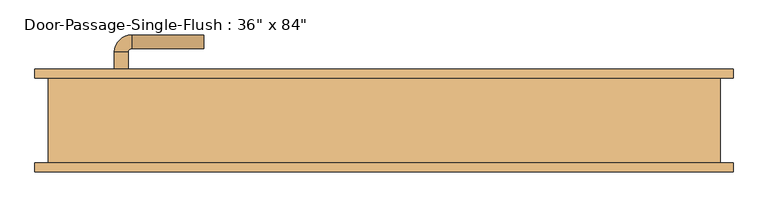
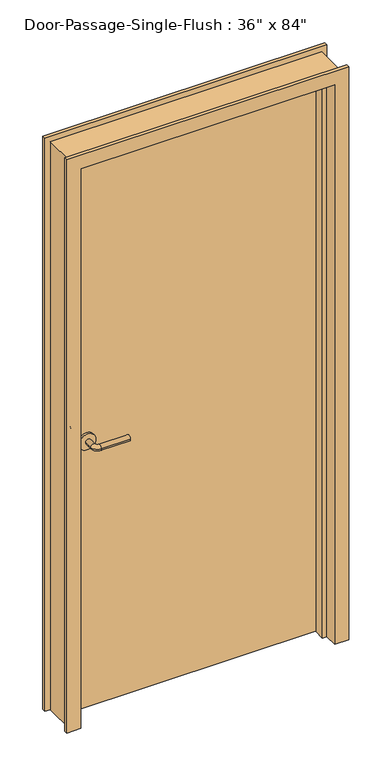
"""IFC4 building model written with IfcOpenShell, lengths in millimetres: door geometry."""

import ifcopenshell
import ifcopenshell.guid

model = None  # the IFC model being written
_history = None  # IfcOwnerHistory: only IFC2X3 demands one
_inside = {}  # id of a spatial element -> (the spatial element, [elements in it])
_under = {}  # id of a project, library or spatial element -> (it, [spatial elements below it])
_declared = {}  # id of a project -> (the project, [libraries it declares])
_typed = {}  # id of a type object -> (the type object, [elements of that type])
_made_of = {}  # id of a material, layer set ... -> (it, [elements and type objects made of it])


def new_model(schema):
    """Start an empty IFC model of exactly this schema.

    Asked for "IFC4X3", IfcOpenShell would pick the latest addendum, in which some entities
    have other attributes; the version numbers below select the first issue.
    IFC2X3 requires an IfcOwnerHistory on every rooted entity: one is made here for all.
    """
    global model, _history
    if schema == "IFC4X3":
        model = ifcopenshell.file(schema_version=(4, 3, 0, 0))
    else:
        model = ifcopenshell.file(schema=schema)
    _inside.clear()
    _under.clear()
    _declared.clear()
    _typed.clear()
    _made_of.clear()
    _history = None
    if model.schema == "IFC2X3":
        org = make("IfcOrganization", Name="unknown")
        user = make(
            "IfcPersonAndOrganization",
            ThePerson=make("IfcPerson", FamilyName="unknown"),
            TheOrganization=org,
        )
        app = make(
            "IfcApplication",
            ApplicationDeveloper=org,
            Version="unknown",
            ApplicationFullName="unknown",
            ApplicationIdentifier="unknown",
        )
        _history = make(
            "IfcOwnerHistory",
            OwningUser=user,
            OwningApplication=app,
            ChangeAction="ADDED",
            CreationDate=0,
        )
    return model


def make(cls, **values):
    """One entity of the class cls with the attributes given. An attribute that is None is left unset."""
    return model.create_entity(
        cls, **{name: value for name, value in values.items() if value is not None}
    )


def rooted(cls, **values):
    """An entity with a GlobalId (a new one), such as an element, a storey or a relation."""
    return make(cls, GlobalId=ifcopenshell.guid.new(), OwnerHistory=_history, **values)


def si_unit(unit_type, name, prefix=None):
    """IfcSIUnit, for example si_unit("LENGTHUNIT", "METRE", prefix="MILLI")."""
    return make("IfcSIUnit", UnitType=unit_type, Prefix=prefix, Name=name)


def assignment(units):
    """IfcUnitAssignment: the units of a project."""
    return None if units is None else make("IfcUnitAssignment", Units=units)


def point(xyz):
    """IfcCartesianPoint."""
    return None if xyz is None else make("IfcCartesianPoint", Coordinates=xyz)


def direction(xyz):
    """IfcDirection."""
    return None if xyz is None else make("IfcDirection", DirectionRatios=xyz)


def frame(location, z_axis=None, x_axis=None):
    """IfcAxis2Placement3D, a coordinate frame: its origin and axes. An axis left out is left unset."""
    return make(
        "IfcAxis2Placement3D",
        Location=point(location),
        Axis=direction(z_axis),
        RefDirection=direction(x_axis),
    )


def frame_2d(location, x_axis=None):
    """IfcAxis2Placement2D, a coordinate frame in the plane: its origin and x axis."""
    return make(
        "IfcAxis2Placement2D", Location=point(location), RefDirection=direction(x_axis)
    )


def origin():
    """The frame at (0, 0, 0) with its axes left unset."""
    return frame((0.0, 0.0, 0.0))


def origin_with_axes():
    """The frame at (0, 0, 0) with the z axis (0, 0, 1) and the x axis (1, 0, 0) written out."""
    return frame((0.0, 0.0, 0.0), z_axis=(0.0, 0.0, 1.0), x_axis=(1.0, 0.0, 0.0))


def place(relative_to, where):
    """IfcLocalPlacement: puts the frame where relative to a parent placement (None: the world)."""
    return make(
        "IfcLocalPlacement", PlacementRelTo=relative_to, RelativePlacement=where
    )


def context(
    kind, dimensions, precision=None, world=None, true_north=None, identifier=None
):
    """IfcGeometricRepresentationContext, for example the 3D "Model" context."""
    return make(
        "IfcGeometricRepresentationContext",
        ContextIdentifier=identifier,
        ContextType=kind,
        CoordinateSpaceDimension=dimensions,
        Precision=precision,
        WorldCoordinateSystem=world,
        TrueNorth=true_north,
    )


def project(units=None, contexts=None):
    """IfcProject with its units and contexts."""
    return rooted(
        "IfcProject",
        Name="project",
        RepresentationContexts=contexts,
        UnitsInContext=assignment(units),
    )


def spatial(cls, under=None, at=None, **own):
    """A site, building, storey or space (cls), placed at a placement, below another one or the project."""
    s = rooted(cls, ObjectPlacement=at, **own)
    if under is not None:
        _under.setdefault(under.id(), (under, []))[1].append(s)
    return s


def polyline(points):
    """IfcPolyline through the points."""
    return make("IfcPolyline", Points=[point(p) for p in points])


def circle_curve(where, radius):
    """IfcCircle in the frame where."""
    return make("IfcCircle", Position=where, Radius=radius)


def ellipse_curve(where, semi_axis1, semi_axis2):
    """IfcEllipse in the frame where."""
    return make(
        "IfcEllipse", Position=where, SemiAxis1=semi_axis1, SemiAxis2=semi_axis2
    )


def trimmed(basis, trim1, trim2, sense, master):
    """IfcTrimmedCurve: the piece of a basis curve between two trims."""
    return make(
        "IfcTrimmedCurve",
        BasisCurve=basis,
        Trim1=trim1,
        Trim2=trim2,
        SenseAgreement=sense,
        MasterRepresentation=master,
    )


def segment(curve, same_sense, transition):
    """IfcCompositeCurveSegment."""
    return make(
        "IfcCompositeCurveSegment",
        Transition=transition,
        SameSense=same_sense,
        ParentCurve=curve,
    )


def composite_curve(segments, self_intersect=None):
    """IfcCompositeCurve: segments joined end to end."""
    return make("IfcCompositeCurve", Segments=segments, SelfIntersect=self_intersect)


def outline(outer, holes=None, kind="AREA"):
    """IfcArbitraryClosedProfileDef: a profile drawn as a closed curve; with holes, ...WithVoids."""
    if holes is None:
        return make("IfcArbitraryClosedProfileDef", ProfileType=kind, OuterCurve=outer)
    return make(
        "IfcArbitraryProfileDefWithVoids",
        ProfileType=kind,
        OuterCurve=outer,
        InnerCurves=holes,
    )


def extrude(swept, where, along, depth):
    """IfcExtrudedAreaSolid: the profile swept, set in the frame where, extruded along a direction by depth."""
    return make(
        "IfcExtrudedAreaSolid",
        SweptArea=swept,
        Position=where,
        ExtrudedDirection=direction(along),
        Depth=depth,
    )


def faces_of(points, faces, orient=None, outer=None):
    """IfcFace entities. A face is a list of loops; a loop is a list of indices into points, from 0.

    orient and outer hold one flag for each loop. By default every Orientation is true, the
    first loop of a face is its IfcFaceOuterBound and the others are IfcFaceBound.
    """
    made = []
    for i, loops in enumerate(faces):
        bounds = []
        for j, loop in enumerate(loops):
            is_outer = j == 0 if outer is None else outer[i][j]
            bounds.append(
                make(
                    "IfcFaceOuterBound" if is_outer else "IfcFaceBound",
                    Bound=make("IfcPolyLoop", Polygon=[points[k] for k in loop]),
                    Orientation=True if orient is None else orient[i][j],
                )
            )
        made.append(make("IfcFace", Bounds=bounds))
    return made


def faceted_brep(points, faces, orient=None, outer=None, voids=None):
    """IfcFacetedBrep: a solid bounded by flat faces; with voids (closed shells), ...WithVoids."""
    shared = [point(p) for p in points]
    hull = make("IfcClosedShell", CfsFaces=faces_of(shared, faces, orient, outer))
    if voids is None:
        return make("IfcFacetedBrep", Outer=hull)
    return make(
        "IfcFacetedBrepWithVoids",
        Outer=hull,
        Voids=[
            make(cls, CfsFaces=faces_of(shared, fs, o, b)) for cls, fs, o, b in voids
        ],
    )


def shape(context_of_items, identifier, shape_type, items):
    """IfcShapeRepresentation: the items that make up one representation, for example the "Body"."""
    return make(
        "IfcShapeRepresentation",
        ContextOfItems=context_of_items,
        RepresentationIdentifier=identifier,
        RepresentationType=shape_type,
        Items=items,
    )


def source(mapping_origin, context_of_items, identifier, shape_type, items):
    """IfcRepresentationMap: a shape defined once, which mapped items show again and again."""
    return make(
        "IfcRepresentationMap",
        MappingOrigin=mapping_origin,
        MappedRepresentation=shape(context_of_items, identifier, shape_type, items),
    )


def transform(
    local_origin,
    x_axis=None,
    y_axis=None,
    z_axis=None,
    scale=None,
    scale2=None,
    scale3=None,
    uniform=True,
):
    """IfcCartesianTransformationOperator3D, or its non-uniform kind. x_axis, y_axis, z_axis: its Axis1, 2, 3."""
    if uniform:
        return make(
            "IfcCartesianTransformationOperator3D",
            Axis1=direction(x_axis),
            Axis2=direction(y_axis),
            LocalOrigin=point(local_origin),
            Scale=scale,
            Axis3=direction(z_axis),
        )
    return make(
        "IfcCartesianTransformationOperator3DnonUniform",
        Axis1=direction(x_axis),
        Axis2=direction(y_axis),
        LocalOrigin=point(local_origin),
        Scale=scale,
        Axis3=direction(z_axis),
        Scale2=scale2,
        Scale3=scale3,
    )


def mapped(mapping_source, mapping_target):
    """IfcMappedItem: shows the shape of a source again, moved by a transform."""
    return make(
        "IfcMappedItem", MappingSource=mapping_source, MappingTarget=mapping_target
    )


def made_of(thing, what):
    """Note that an element or type object is made of a material, layer set ...; save() writes the relation."""
    if what is not None:
        _made_of.setdefault(what.id(), (what, []))[1].append(thing)
    return thing


def element(
    cls,
    number,
    at=None,
    inside=None,
    cuts=None,
    type_object=None,
    material=None,
    context=None,
    identifier="Body",
    shape_type=None,
    held_by="IfcProductDefinitionShape",
    body=None,
    shapes=None,
    **own,
):
    """One element of the class cls, such as IfcWall. Its Tag is "e" and its number.

    at: its placement. inside: the storey or other place that contains it. cuts: it is an
    opening in that element (IfcRelVoidsElement). A single representation is given by context,
    identifier, shape_type and body (its items); several are given by shapes. held_by: the class
    of the entity that holds the representations. save() writes the other relations.
    """
    e = rooted(cls, Tag="e%d" % number, ObjectPlacement=at, **own)
    if body is not None:
        shapes = [shape(context, identifier, shape_type, body)]
    if shapes is not None:
        e.Representation = make(held_by, Representations=shapes)
    if inside is not None:
        _inside.setdefault(inside.id(), (inside, []))[1].append(e)
    if cuts is not None:
        rooted(
            "IfcRelVoidsElement", RelatingBuildingElement=cuts, RelatedOpeningElement=e
        )
    if type_object is not None:
        _typed.setdefault(type_object.id(), (type_object, []))[1].append(e)
    return made_of(e, material)


def aggregate(whole, parts):
    """IfcRelAggregates: a whole, such as a stair, and the parts it consists of."""
    return rooted("IfcRelAggregates", RelatingObject=whole, RelatedObjects=parts)


def save(model, path):
    """Write the relations noted so far, then the file.

    IfcRelAggregates (storeys below a building ...), IfcRelContainedInSpatialStructure (elements
    in a storey), IfcRelDefinesByType, IfcRelAssociatesMaterial and IfcRelDeclares: one each for
    every whole, place, type object, material and project.
    """
    for whole, parts in _under.values():
        aggregate(whole, parts)
    for where, things in _inside.values():
        rooted(
            "IfcRelContainedInSpatialStructure",
            RelatedElements=things,
            RelatingStructure=where,
        )
    for kind, things in _typed.values():
        rooted("IfcRelDefinesByType", RelatedObjects=things, RelatingType=kind)
    for what, things in _made_of.values():
        rooted("IfcRelAssociatesMaterial", RelatedObjects=things, RelatingMaterial=what)
    for by, libraries in _declared.values():
        rooted("IfcRelDeclares", RelatingContext=by, RelatedDefinitions=libraries)
    model.write(path)


def plane_surface(at):
    """IfcPlane: the flat surface through the origin of the frame at, square to its z axis."""
    return make("IfcPlane", Position=at)


def cylinder_surface(at, radius):
    """IfcCylindricalSurface: all points at the distance radius from the z axis of the frame at."""
    return make("IfcCylindricalSurface", Position=at, Radius=radius)


def revolved_surface(curve, axis_point, axis_direction):
    """IfcSurfaceOfRevolution: the curve turned about the line through axis_point along axis_direction."""
    return make(
        "IfcSurfaceOfRevolution",
        SweptCurve=make("IfcArbitraryOpenProfileDef", ProfileType="CURVE", Curve=curve),
        AxisPosition=make("IfcAxis1Placement", Location=point(axis_point), Axis=direction(axis_direction)),
    )


def advanced_brep(points, edges, surfaces, faces):
    """IfcAdvancedBrep: a solid bounded by faces that lie on surfaces and meet in shared edges.

    An edge is (start, end): straight between two places in points (the first is 0);
    or (start, end, curve); or (start, end, curve, False) where it runs against its curve.
    A face is (place in surfaces, loops), or (place, loops, False) where it looks against
    its surface's normal. A loop lists edges by number (the first is 1), with a minus sign
    where the edge is run from its end to its start. The first loop is the outer one.
    """
    corners = [point(p) for p in points]
    vertices = [make("IfcVertexPoint", VertexGeometry=c) for c in corners]
    made = []
    for start, end, *more in edges:
        made.append(
            make(
                "IfcEdgeCurve",
                EdgeStart=vertices[start],
                EdgeEnd=vertices[end],
                EdgeGeometry=more[0] if more else make("IfcPolyline", Points=[corners[start], corners[end]]),
                SameSense=more[1] if len(more) > 1 else True,
            )
        )
    hull = []
    for where, loops, *sense in faces:
        bounds = []
        for j, loop in enumerate(loops):
            ring = [make("IfcOrientedEdge", EdgeElement=made[abs(k) - 1], Orientation=k > 0) for k in loop]
            bounds.append(
                make(
                    "IfcFaceOuterBound" if j == 0 else "IfcFaceBound",
                    Bound=make("IfcEdgeLoop", EdgeList=ring),
                    Orientation=True,
                )
            )
        hull.append(make("IfcAdvancedFace", Bounds=bounds, FaceSurface=surfaces[where], SameSense=sense[0] if sense else True))
    return make("IfcAdvancedBrep", Outer=make("IfcClosedShell", CfsFaces=hull))


def door_6d6a07ab(model_context):
    return source(origin(), model_context, "Body", "SolidModel", [
        advanced_brep(
        [(-392.190625, 15.8125, 1016.0), (-372.190625, 15.8125, 1016.0), (-372.190625, -14.1875, 1016.0), (-392.190625, -14.1875, 1016.0), (-367.190625, -19.1875, 1016.0), (-367.190625, -39.1875, 1016.0), (-262.190625, -39.1875, 1016.0), (-262.190625, -19.1875, 1016.0)],
        [
            (0, 1, circle_curve(frame((-382.190625, 15.8125, 1016.0), z_axis=(0.0, 1.0, 0.0), x_axis=(1.0, 0.0, 0.0)), 10.0)),
            (1, 0, circle_curve(frame((-382.190625, 15.8125, 1016.0), z_axis=(0.0, 1.0, 0.0), x_axis=(1.0, 0.0, 0.0)), 10.0)),
            (1, 2),
            (2, 3, circle_curve(frame((-382.190625, -14.1875, 1016.0), z_axis=(0.0, 1.0, 0.0), x_axis=(1.0, 0.0, 0.0)), 10.0)),
            (3, 0),
            (3, 2, circle_curve(frame((-382.190625, -14.1875, 1016.0), z_axis=(0.0, 1.0, 0.0), x_axis=(1.0, 0.0, 0.0)), 10.0)),
            (4, 5, circle_curve(frame((-367.190625, -29.1875, 1016.0), z_axis=(-1.0, 0.0, 0.0), x_axis=(0.0, 1.0, 0.0)), 10.0)),
            (5, 3, circle_curve(frame((-367.190625, -14.1875, 1016.0), z_axis=(0.0, 0.0, -1.0), x_axis=(-1.0, 0.0, 0.0)), 25.0)),
            (2, 4, circle_curve(frame((-367.190625, -14.1875, 1016.0), z_axis=(0.0, 0.0, 1.0), x_axis=(-1.0, 0.0, 0.0)), 5.0)),
            (5, 4, circle_curve(frame((-367.190625, -29.1875, 1016.0), z_axis=(-1.0, 0.0, 0.0), x_axis=(0.0, 1.0, 0.0)), 10.0)),
            (6, 7, circle_curve(frame((-262.190625, -29.1875, 1016.0), z_axis=(1.0, 0.0, 0.0), x_axis=(0.0, 1.0, 0.0)), 10.0)),
            (7, 6, circle_curve(frame((-262.190625, -29.1875, 1016.0), z_axis=(1.0, 0.0, 0.0), x_axis=(0.0, 1.0, 0.0)), 10.0)),
            (4, 7),
            (6, 5),
        ],
        [
            plane_surface(frame((-382.190625, 15.8125, 1016.0), z_axis=(0.0, 1.0, 0.0), x_axis=(0.0, 0.0, 1.0))),
            cylinder_surface(frame((-382.190625, 15.8125, 1016.0), z_axis=(0.0, 1.0, 0.0), x_axis=(1.0, 0.0, 0.0)), 10.0),
            revolved_surface(trimmed(ellipse_curve(frame((-382.190625, -14.1875, 1016.0), z_axis=(0.0, -1.0, 0.0), x_axis=(1.0, 0.0, 0.0)), 10.0, 10.0), [point((-392.190625, -14.1875, 1016.0))], [point((-372.190625, -14.1875, 1016.0))], True, "CARTESIAN"), (-367.190625, -14.1875, 1016.0), (0.0, 0.0, -1.0)),
            revolved_surface(trimmed(ellipse_curve(frame((-382.190625, -14.1875, 1016.0), z_axis=(0.0, -1.0, 0.0), x_axis=(1.0, 0.0, 0.0)), 10.0, 10.0), [point((-372.190625, -14.1875, 1016.0))], [point((-392.190625, -14.1875, 1016.0))], True, "CARTESIAN"), (-367.190625, -14.1875, 1016.0), (0.0, 0.0, -1.0)),
            plane_surface(frame((-262.190625, -29.1875, 1016.0), z_axis=(1.0, 0.0, 0.0), x_axis=(0.0, 0.0, 1.0))),
            cylinder_surface(frame((-367.190625, -29.1875, 1016.0), z_axis=(-1.0, 0.0, 0.0), x_axis=(0.0, 1.0, 0.0)), 10.0),
        ],
        [
            (0, [[1, 2]]),
            (1, [[3, 4, 5, -2]]),
            (1, [[-5, 6, -3, -1]]),
            (2, [[7, 8, -4, 9]]),
            (3, [[10, -9, -6, -8]]),
            (4, [[11, 12]]),
            (5, [[13, -11, 14, -7]]),
            (5, [[-14, -12, -13, -10]]),
        ],
    ),
        extrude(outline(composite_curve([segment(trimmed(circle_curve(frame_2d((1016.0, -384.690625)), 30.0), [point((1016.0, -414.690625))], [point((1016.0, -354.690625))], False, "CARTESIAN"), True, "CONTINUOUS"), segment(trimmed(circle_curve(frame_2d((1016.0, -384.690625)), 30.0), [point((1016.0, -354.690625))], [point((1016.0, -414.690625))], False, "CARTESIAN"), True, "CONTINUOUS")], self_intersect=False)), frame((0.0, 15.8125, 0.0), z_axis=(0.0, 1.0, 0.0), x_axis=(0.0, 0.0, 1.0)), (0.0, 0.0, 1.0), 8.0),
        advanced_brep(
        [(-392.190625, 76.2625, 1016.0), (-372.190625, 76.2625, 1016.0), (-392.190625, 106.2625, 1016.0), (-372.190625, 106.2625, 1016.0), (-367.190625, 111.2625, 1016.0), (-367.190625, 131.2625, 1016.0), (-262.190625, 131.2625, 1016.0), (-262.190625, 111.2625, 1016.0)],
        [
            (0, 1, circle_curve(frame((-382.190625, 76.2625, 1016.0), z_axis=(0.0, -1.0, 0.0), x_axis=(1.0, 0.0, 0.0)), 10.0)),
            (1, 0, circle_curve(frame((-382.190625, 76.2625, 1016.0), z_axis=(0.0, -1.0, 0.0), x_axis=(1.0, 0.0, 0.0)), 10.0)),
            (0, 2),
            (2, 3, circle_curve(frame((-382.190625, 106.2625, 1016.0), z_axis=(0.0, -1.0, 0.0), x_axis=(1.0, 0.0, 0.0)), 10.0)),
            (3, 1),
            (3, 2, circle_curve(frame((-382.190625, 106.2625, 1016.0), z_axis=(0.0, -1.0, 0.0), x_axis=(1.0, 0.0, 0.0)), 10.0)),
            (4, 3, circle_curve(frame((-367.190625, 106.2625, 1016.0), z_axis=(0.0, 0.0, 1.0), x_axis=(-1.0, 0.0, 0.0)), 5.0)),
            (2, 5, circle_curve(frame((-367.190625, 106.2625, 1016.0), z_axis=(0.0, 0.0, -1.0), x_axis=(-1.0, 0.0, 0.0)), 25.0)),
            (5, 4, circle_curve(frame((-367.190625, 121.2625, 1016.0), z_axis=(-1.0, 0.0, 0.0), x_axis=(0.0, -1.0, 0.0)), 10.0)),
            (4, 5, circle_curve(frame((-367.190625, 121.2625, 1016.0), z_axis=(-1.0, 0.0, 0.0), x_axis=(0.0, -1.0, 0.0)), 10.0)),
            (6, 7, circle_curve(frame((-262.190625, 121.2625, 1016.0), z_axis=(1.0, 0.0, 0.0), x_axis=(0.0, -1.0, 0.0)), 10.0)),
            (7, 6, circle_curve(frame((-262.190625, 121.2625, 1016.0), z_axis=(1.0, 0.0, 0.0), x_axis=(0.0, -1.0, 0.0)), 10.0)),
            (5, 6),
            (7, 4),
        ],
        [
            plane_surface(frame((-382.190625, 76.2625, 1016.0), z_axis=(0.0, -1.0, 0.0), x_axis=(0.0, 0.0, 1.0))),
            cylinder_surface(frame((-382.190625, 76.2625, 1016.0), z_axis=(0.0, -1.0, 0.0), x_axis=(1.0, 0.0, 0.0)), 10.0),
            revolved_surface(trimmed(ellipse_curve(frame((-382.190625, 106.2625, 1016.0), z_axis=(0.0, -1.0, 0.0), x_axis=(1.0, 0.0, 0.0)), 10.0, 10.0), [point((-392.190625, 106.2625, 1016.0))], [point((-372.190625, 106.2625, 1016.0))], True, "CARTESIAN"), (-367.190625, 106.2625, 1016.0), (0.0, 0.0, -1.0)),
            revolved_surface(trimmed(ellipse_curve(frame((-382.190625, 106.2625, 1016.0), z_axis=(0.0, -1.0, 0.0), x_axis=(1.0, 0.0, 0.0)), 10.0, 10.0), [point((-372.190625, 106.2625, 1016.0))], [point((-392.190625, 106.2625, 1016.0))], True, "CARTESIAN"), (-367.190625, 106.2625, 1016.0), (0.0, 0.0, -1.0)),
            plane_surface(frame((-262.190625, 121.2625, 1016.0), z_axis=(1.0, 0.0, 0.0), x_axis=(0.0, 0.0, 1.0))),
            cylinder_surface(frame((-367.190625, 121.2625, 1016.0), z_axis=(-1.0, 0.0, 0.0), x_axis=(0.0, -1.0, 0.0)), 10.0),
        ],
        [
            (0, [[1, 2]]),
            (1, [[-1, 3, 4, 5]]),
            (1, [[-2, -5, 6, -3]]),
            (2, [[7, -4, 8, 9]]),
            (3, [[-8, -6, -7, 10]]),
            (4, [[11, 12]]),
            (5, [[-9, 13, -12, 14]]),
            (5, [[-10, -14, -11, -13]]),
        ],
    ),
        extrude(outline(composite_curve([segment(trimmed(circle_curve(frame_2d((1016.0, -384.690625)), 30.0), [point((1016.0, -414.690625))], [point((1016.0, -354.690625))], False, "CARTESIAN"), True, "CONTINUOUS"), segment(trimmed(circle_curve(frame_2d((1016.0, -384.690625)), 30.0), [point((1016.0, -354.690625))], [point((1016.0, -414.690625))], False, "CARTESIAN"), True, "CONTINUOUS")], self_intersect=False)), frame((0.0, 68.2625, 0.0), z_axis=(0.0, 1.0, 0.0), x_axis=(0.0, 0.0, 1.0)), (0.0, 0.0, 1.0), 8.0),
        faceted_brep([(457.2, 80.9625, 0.0), (508.0, 80.9625, 0.0), (508.0, 68.2625, 0.0), (488.95, 68.2625, 0.0), (488.95, -55.5625, 0.0), (508.0, -55.5625, 0.0), (508.0, -68.2625, 0.0), (457.2, -68.2625, 0.0), (457.2, -19.05, 0.0), (441.325, -19.05, 0.0), (441.325, 19.05, 0.0), (457.2, 19.05, 0.0), (457.2, 80.9625, 2133.6), (-457.2, 80.9625, 2133.6), (-457.2, 80.9625, 0.0), (-508.0, 80.9625, 0.0), (-508.0, 80.9625, 2184.4), (508.0, 80.9625, 2184.4), (508.0, 68.2625, 2184.4), (-508.0, 68.2625, 2184.4), (-508.0, 68.2625, 0.0), (-488.95, 68.2625, 0.0), (-488.95, 68.2625, 2165.35), (488.95, 68.2625, 2165.35), (488.95, -55.5625, 2165.35), (-488.95, -55.5625, 2165.35), (-488.95, -55.5625, 0.0), (-508.0, -55.5625, 0.0), (-508.0, -55.5625, 2184.4), (508.0, -55.5625, 2184.4), (508.0, -68.2625, 2184.4), (-508.0, -68.2625, 2184.4), (-508.0, -68.2625, 0.0), (-457.2, -68.2625, 0.0), (-457.2, -68.2625, 2133.6), (457.2, -68.2625, 2133.6), (457.2, -19.05, 2133.6), (-457.2, -19.05, 2133.6), (-457.2, -19.05, 0.0), (-441.325, -19.05, 0.0), (-441.325, -19.05, 2117.725), (441.325, -19.05, 2117.725), (441.325, 19.05, 2117.725), (-441.325, 19.05, 2117.725), (-441.325, 19.05, 0.0), (-457.2, 19.05, 0.0), (-457.2, 19.05, 2133.6), (457.2, 19.05, 2133.6)], [[[0, 1, 2, 3, 4, 5, 6, 7, 8, 9, 10, 11]], [[1, 0, 12, 13, 14, 15, 16, 17]], [[2, 1, 17, 18]], [[3, 2, 18, 19, 20, 21, 22, 23]], [[4, 3, 23, 24]], [[5, 4, 24, 25, 26, 27, 28, 29]], [[6, 5, 29, 30]], [[7, 6, 30, 31, 32, 33, 34, 35]], [[8, 7, 35, 36]], [[9, 8, 36, 37, 38, 39, 40, 41]], [[10, 9, 41, 42]], [[11, 10, 42, 43, 44, 45, 46, 47]], [[0, 11, 47, 12]], [[18, 17, 16, 19]], [[24, 23, 22, 25]], [[30, 29, 28, 31]], [[36, 35, 34, 37]], [[42, 41, 40, 43]], [[12, 47, 46, 13]], [[14, 45, 44, 39, 38, 33, 32, 27, 26, 21, 20, 15]], [[19, 16, 15, 20]], [[25, 22, 21, 26]], [[31, 28, 27, 32]], [[37, 34, 33, 38]], [[43, 40, 39, 44]], [[13, 46, 45, 14]]]),
        extrude(outline(polyline([(457.2, 23.8125), (-457.2, 23.8125), (-457.2, 68.2625), (457.2, 68.2625), (457.2, 23.8125)])), origin_with_axes(), (0.0, 0.0, 1.0), 2133.6),
    ])


if __name__ == "__main__":
    model = new_model("IFC4")
    model_context = context("Model", 3, world=origin())
    ifc_project = project(units=[si_unit("LENGTHUNIT", "METRE", prefix="MILLI")], contexts=[model_context])
    site = spatial("IfcSite", under=ifc_project)
    building = spatial("IfcBuilding", under=site)
    placement = place(None, origin())
    door_shape = door_6d6a07ab(model_context)
    element("IfcDoor", 1, ObjectType="Door-Passage-Single-Flush : 36\" x 84\"", at=placement, inside=building, context=model_context, shape_type="MappedRepresentation", body=[
        mapped(door_shape, transform((0.0, 0.0, 0.0), x_axis=(1.0, 0.0, 0.0), y_axis=(0.0, 1.0, 0.0), z_axis=(0.0, 0.0, 1.0))),
    ])
    save(model, "model.ifc")

# Revit data of these elements
# Type "Door-Passage-Single-Flush : 36\" x 84\""
#   Type Mark = "1"
#   Assembly Code = "B2030200"
#   Analytic Construction = "Wooden"
#   Thickness = 0' - 1 3/4"
#   Thermal Resistance (R) = 2.5876 (h·ft²·°F)/BTU
#   Swing Angle [instance default] = 90.00°
#   Strike Height = 3' - 4"
#   Rough Width [instance default] = 3' - 4"
#   Rough Height [instance default] = 7' - 4"
#   MF Opening Height [instance default] = 0' - 4"
#   MF Opening Width [instance default] = 0' - 4"
#   Inset Calculate [instance default] = 0' - 4"
#   Masonry Inset [instance default] = 0' - 1"
#   Height = 7' - 0"
#   Width = 3' - 0"
#   Heat Transfer Coefficient (U) = 0.3865 BTU/(h·ft²·°F)
#   Masonry Frame Depth = 0' - 5 3/4"
#   Define Thermal Properties by = 1
#   Masonry Frame [instance default] = yes
#   Function = 1
#   Dry Wall Frame [instance default] = no
#   Panel Material = Wood - Birch
#   Frame Material = Metal - Paint Finish - Grey
#   Door Handle Material = Aluminum
#   Visual Light Transmittance = 0
#   Solar Heat Gain Coefficient = 0
#   Wall Closure = (empty or 0)
# Element 1 (IfcDoor, "Door-Passage-Single-Flush : 36\" x 84\"")
#   Rough Width = 3' - 2 1/2"
#   Rough Height = 7' - 1 1/4"
#   MF Opening Height = 0' - 1 1/4"
#   MF Opening Width = 0' - 2 1/2"
#   Inset Calculate = 0' - 3"
#   Masonry Frame = no
#   Dry Wall Frame = yes
#   Materials on its faces: "Metal - Paint Finish - Grey", "Aluminum", "Wood - Birch"
# Materials
#   "Wood - Birch": class "Wood", colour RGB 166 116 52, transparency 0, Cost = 0
#   "Metal - Paint Finish - Grey": class "Paint", colour RGB 104 104 104, transparency 0, Cost = 0
#   "Aluminum": class "Metal", colour RGB 247 247 247, transparency 0, Description = "Aluminum 6061", Cost = 0
